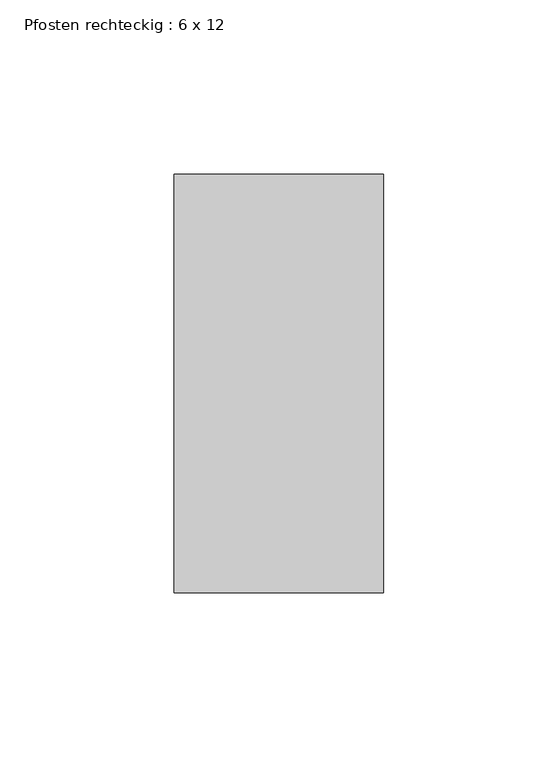
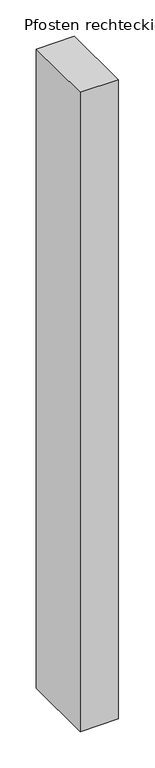
"""IFC4 building model written with IfcOpenShell, lengths in millimetres: member geometry, Pfosten rechteckig : 6 x 12."""

from ifc_helpers import new_model, si_unit, frame, origin, place, context, project, spatial, polyline, outline, extrude, source, transform, mapped, element, save


def pfosten_rechteckig_6_x_12_9b31b77d(model_context):
    return source(origin(), model_context, "Body", "SweptSolid", [
        extrude(outline(polyline([(30.0, 60.0), (30.0, -60.0), (-30.0, -60.0), (-30.0, 60.0), (30.0, 60.0)])), frame((0.0, 0.0, -1069.9773049), z_axis=(0.0, 0.0, 1.0), x_axis=(1.0, 0.0, 0.0)), (0.0, 0.0, 1.0), 1069.9773049),
    ])


if __name__ == "__main__":
    model = new_model("IFC4")
    model_context = context("Model", 3, world=origin())
    ifc_project = project(units=[si_unit("LENGTHUNIT", "METRE", prefix="MILLI")], contexts=[model_context])
    site = spatial("IfcSite", under=ifc_project)
    building = spatial("IfcBuilding", under=site)
    placement = place(None, origin())
    pfosten_rechteckig_6_x_12_shape = pfosten_rechteckig_6_x_12_9b31b77d(model_context)
    element("IfcMember", 1, ObjectType="Pfosten rechteckig : 6 x 12", at=placement, inside=building, context=model_context, shape_type="MappedRepresentation", body=[
        mapped(pfosten_rechteckig_6_x_12_shape, transform((0.0, 0.0, 0.0), x_axis=(1.0, 0.0, 0.0), y_axis=(0.0, 1.0, 0.0), z_axis=(0.0, 0.0, 1.0))),
    ])
    save(model, "model.ifc")

# Revit data of these elements
# Type "Pfosten rechteckig : 6 x 12"
#   built-in parameter 1007304 = 0.393701 (stored number, unit not read)
#   built-in parameter 1007301 = 0.0984252 (stored number, unit not read)
#   built-in parameter 1007300 = 0.0984252 (stored number, unit not read)
# Element 1 (IfcMember, "Pfosten rechteckig : 6 x 12")
#   Materials on its faces: "Metall - verzinkt"
# Materials
#   "Metall - verzinkt": class "Allgemeines", colour RGB 200 200 200, transparency 0, Cost = 0
